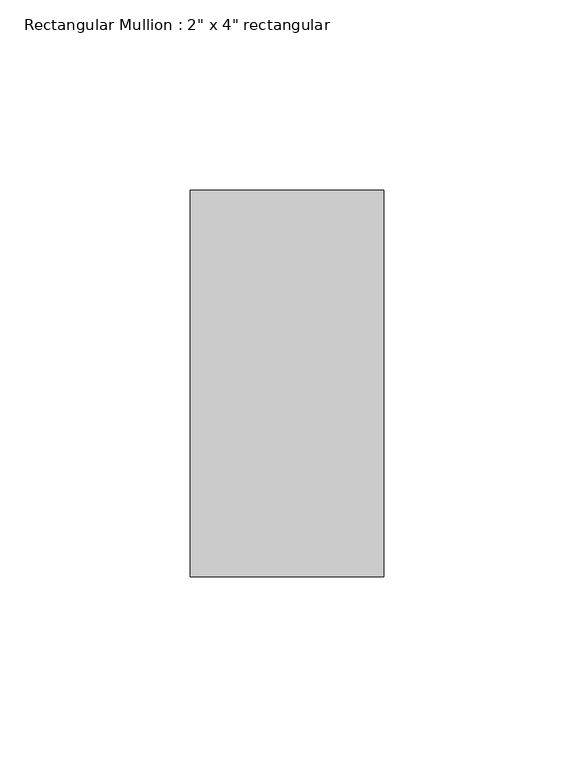
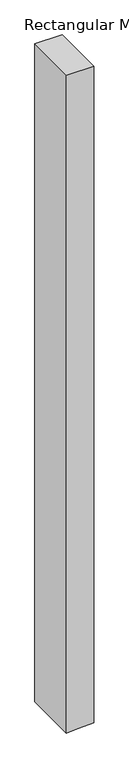
"""IFC4 building model written with IfcOpenShell, lengths in millimetres: member geometry."""

from ifc_helpers import new_model, si_unit, frame, origin, place, context, project, spatial, polyline, outline, extrude, source, transform, mapped, element, save


def member_081ce7d1(model_context):
    return source(origin(), model_context, "Body", "SweptSolid", [
        extrude(outline(polyline([(0.0, 25.4), (0.0, -25.4), (-1294.9266526, -25.4), (-1293.9564372, -2.1148317), (-1292.8099859, 25.4), (0.0, 25.4)])), frame((0.0, -50.8, 0.0), z_axis=(0.0, 1.0, 0.0), x_axis=(0.0, 0.0, 1.0)), (0.0, 0.0, 1.0), 101.6),
    ])


if __name__ == "__main__":
    model = new_model("IFC4")
    model_context = context("Model", 3, world=origin())
    ifc_project = project(units=[si_unit("LENGTHUNIT", "METRE", prefix="MILLI")], contexts=[model_context])
    site = spatial("IfcSite", under=ifc_project)
    building = spatial("IfcBuilding", under=site)
    placement = place(None, origin())
    member_shape = member_081ce7d1(model_context)
    element("IfcMember", 1, ObjectType="Rectangular Mullion : 2\" x 4\" rectangular", at=placement, inside=building, context=model_context, shape_type="MappedRepresentation", body=[
        mapped(member_shape, transform((0.0, 0.0, 0.0), x_axis=(1.0, 0.0, 0.0), y_axis=(0.0, 1.0, 0.0), z_axis=(0.0, 0.0, 1.0))),
    ])
    save(model, "model.ifc")

# Revit data of these elements
# Type "Rectangular Mullion : 2\" x 4\" rectangular"
#   built-in parameter 1007304 = 0.333333 (stored number, unit not read)
#   built-in parameter 1007301 = 0.0833333 (stored number, unit not read)
#   built-in parameter 1007300 = 0.0833333 (stored number, unit not read)
# Element 1 (IfcMember, "Rectangular Mullion : 2\" x 4\" rectangular")
#   Materials on its faces: "PAINTED STEEL C CHANNEL"
# Materials
#   "PAINTED STEEL C CHANNEL": class "Generic", colour RGB 88 62 61, transparency 0, Cost = 0
